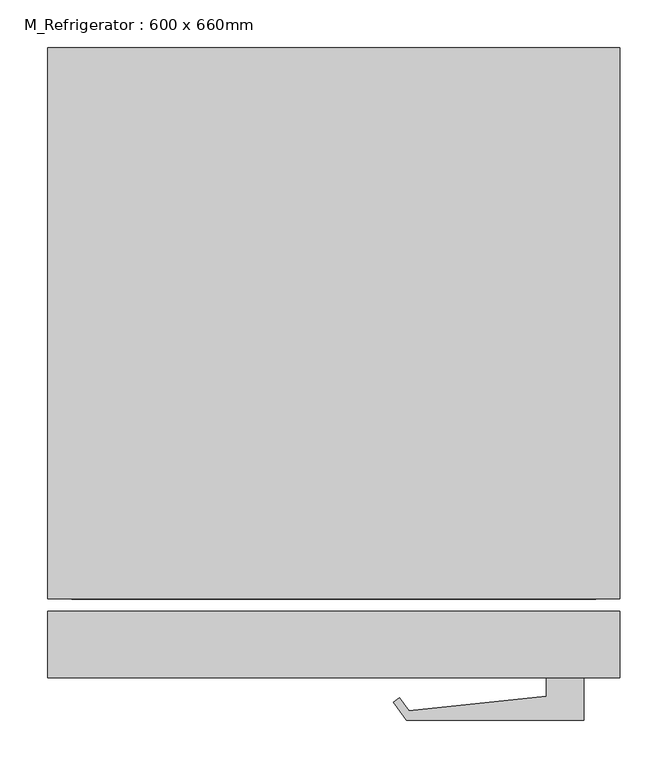
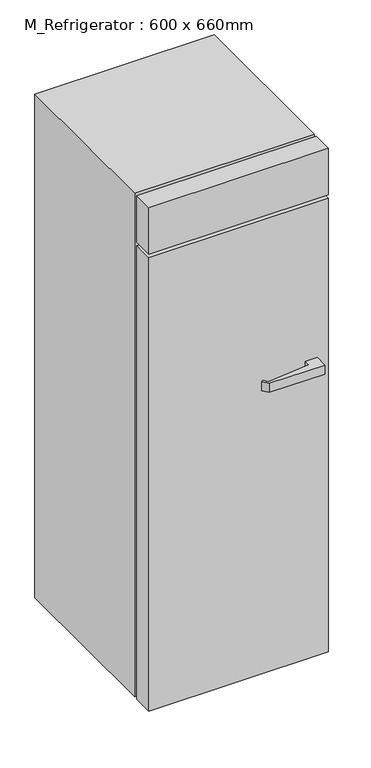
"""IFC4 building model written with IfcOpenShell, lengths in millimetres: proxy geometry, M_Refrigerator : 600 x 660mm."""

import ifcopenshell
import ifcopenshell.guid

model = None  # the IFC model being written
_history = None  # IfcOwnerHistory: only IFC2X3 demands one
_inside = {}  # id of a spatial element -> (the spatial element, [elements in it])
_under = {}  # id of a project, library or spatial element -> (it, [spatial elements below it])
_declared = {}  # id of a project -> (the project, [libraries it declares])
_typed = {}  # id of a type object -> (the type object, [elements of that type])
_made_of = {}  # id of a material, layer set ... -> (it, [elements and type objects made of it])


def new_model(schema):
    """Start an empty IFC model of exactly this schema.

    Asked for "IFC4X3", IfcOpenShell would pick the latest addendum, in which some entities
    have other attributes; the version numbers below select the first issue.
    IFC2X3 requires an IfcOwnerHistory on every rooted entity: one is made here for all.
    """
    global model, _history
    if schema == "IFC4X3":
        model = ifcopenshell.file(schema_version=(4, 3, 0, 0))
    else:
        model = ifcopenshell.file(schema=schema)
    _inside.clear()
    _under.clear()
    _declared.clear()
    _typed.clear()
    _made_of.clear()
    _history = None
    if model.schema == "IFC2X3":
        org = make("IfcOrganization", Name="unknown")
        user = make(
            "IfcPersonAndOrganization",
            ThePerson=make("IfcPerson", FamilyName="unknown"),
            TheOrganization=org,
        )
        app = make(
            "IfcApplication",
            ApplicationDeveloper=org,
            Version="unknown",
            ApplicationFullName="unknown",
            ApplicationIdentifier="unknown",
        )
        _history = make(
            "IfcOwnerHistory",
            OwningUser=user,
            OwningApplication=app,
            ChangeAction="ADDED",
            CreationDate=0,
        )
    return model


def make(cls, **values):
    """One entity of the class cls with the attributes given. An attribute that is None is left unset."""
    return model.create_entity(
        cls, **{name: value for name, value in values.items() if value is not None}
    )


def rooted(cls, **values):
    """An entity with a GlobalId (a new one), such as an element, a storey or a relation."""
    return make(cls, GlobalId=ifcopenshell.guid.new(), OwnerHistory=_history, **values)


def si_unit(unit_type, name, prefix=None):
    """IfcSIUnit, for example si_unit("LENGTHUNIT", "METRE", prefix="MILLI")."""
    return make("IfcSIUnit", UnitType=unit_type, Prefix=prefix, Name=name)


def assignment(units):
    """IfcUnitAssignment: the units of a project."""
    return None if units is None else make("IfcUnitAssignment", Units=units)


def point(xyz):
    """IfcCartesianPoint."""
    return None if xyz is None else make("IfcCartesianPoint", Coordinates=xyz)


def direction(xyz):
    """IfcDirection."""
    return None if xyz is None else make("IfcDirection", DirectionRatios=xyz)


def frame(location, z_axis=None, x_axis=None):
    """IfcAxis2Placement3D, a coordinate frame: its origin and axes. An axis left out is left unset."""
    return make(
        "IfcAxis2Placement3D",
        Location=point(location),
        Axis=direction(z_axis),
        RefDirection=direction(x_axis),
    )


def frame_2d(location, x_axis=None):
    """IfcAxis2Placement2D, a coordinate frame in the plane: its origin and x axis."""
    return make(
        "IfcAxis2Placement2D", Location=point(location), RefDirection=direction(x_axis)
    )


def origin():
    """The frame at (0, 0, 0) with its axes left unset."""
    return frame((0.0, 0.0, 0.0))


def origin_with_axes():
    """The frame at (0, 0, 0) with the z axis (0, 0, 1) and the x axis (1, 0, 0) written out."""
    return frame((0.0, 0.0, 0.0), z_axis=(0.0, 0.0, 1.0), x_axis=(1.0, 0.0, 0.0))


def place(relative_to, where):
    """IfcLocalPlacement: puts the frame where relative to a parent placement (None: the world)."""
    return make(
        "IfcLocalPlacement", PlacementRelTo=relative_to, RelativePlacement=where
    )


def context(
    kind, dimensions, precision=None, world=None, true_north=None, identifier=None
):
    """IfcGeometricRepresentationContext, for example the 3D "Model" context."""
    return make(
        "IfcGeometricRepresentationContext",
        ContextIdentifier=identifier,
        ContextType=kind,
        CoordinateSpaceDimension=dimensions,
        Precision=precision,
        WorldCoordinateSystem=world,
        TrueNorth=true_north,
    )


def project(units=None, contexts=None):
    """IfcProject with its units and contexts."""
    return rooted(
        "IfcProject",
        Name="project",
        RepresentationContexts=contexts,
        UnitsInContext=assignment(units),
    )


def spatial(cls, under=None, at=None, **own):
    """A site, building, storey or space (cls), placed at a placement, below another one or the project."""
    s = rooted(cls, ObjectPlacement=at, **own)
    if under is not None:
        _under.setdefault(under.id(), (under, []))[1].append(s)
    return s


def polyline(points):
    """IfcPolyline through the points."""
    return make("IfcPolyline", Points=[point(p) for p in points])


def circle_curve(where, radius):
    """IfcCircle in the frame where."""
    return make("IfcCircle", Position=where, Radius=radius)


def trimmed(basis, trim1, trim2, sense, master):
    """IfcTrimmedCurve: the piece of a basis curve between two trims."""
    return make(
        "IfcTrimmedCurve",
        BasisCurve=basis,
        Trim1=trim1,
        Trim2=trim2,
        SenseAgreement=sense,
        MasterRepresentation=master,
    )


def segment(curve, same_sense, transition):
    """IfcCompositeCurveSegment."""
    return make(
        "IfcCompositeCurveSegment",
        Transition=transition,
        SameSense=same_sense,
        ParentCurve=curve,
    )


def composite_curve(segments, self_intersect=None):
    """IfcCompositeCurve: segments joined end to end."""
    return make("IfcCompositeCurve", Segments=segments, SelfIntersect=self_intersect)


def outline(outer, holes=None, kind="AREA"):
    """IfcArbitraryClosedProfileDef: a profile drawn as a closed curve; with holes, ...WithVoids."""
    if holes is None:
        return make("IfcArbitraryClosedProfileDef", ProfileType=kind, OuterCurve=outer)
    return make(
        "IfcArbitraryProfileDefWithVoids",
        ProfileType=kind,
        OuterCurve=outer,
        InnerCurves=holes,
    )


def extrude(swept, where, along, depth):
    """IfcExtrudedAreaSolid: the profile swept, set in the frame where, extruded along a direction by depth."""
    return make(
        "IfcExtrudedAreaSolid",
        SweptArea=swept,
        Position=where,
        ExtrudedDirection=direction(along),
        Depth=depth,
    )


def shape(context_of_items, identifier, shape_type, items):
    """IfcShapeRepresentation: the items that make up one representation, for example the "Body"."""
    return make(
        "IfcShapeRepresentation",
        ContextOfItems=context_of_items,
        RepresentationIdentifier=identifier,
        RepresentationType=shape_type,
        Items=items,
    )


def source(mapping_origin, context_of_items, identifier, shape_type, items):
    """IfcRepresentationMap: a shape defined once, which mapped items show again and again."""
    return make(
        "IfcRepresentationMap",
        MappingOrigin=mapping_origin,
        MappedRepresentation=shape(context_of_items, identifier, shape_type, items),
    )


def transform(
    local_origin,
    x_axis=None,
    y_axis=None,
    z_axis=None,
    scale=None,
    scale2=None,
    scale3=None,
    uniform=True,
):
    """IfcCartesianTransformationOperator3D, or its non-uniform kind. x_axis, y_axis, z_axis: its Axis1, 2, 3."""
    if uniform:
        return make(
            "IfcCartesianTransformationOperator3D",
            Axis1=direction(x_axis),
            Axis2=direction(y_axis),
            LocalOrigin=point(local_origin),
            Scale=scale,
            Axis3=direction(z_axis),
        )
    return make(
        "IfcCartesianTransformationOperator3DnonUniform",
        Axis1=direction(x_axis),
        Axis2=direction(y_axis),
        LocalOrigin=point(local_origin),
        Scale=scale,
        Axis3=direction(z_axis),
        Scale2=scale2,
        Scale3=scale3,
    )


def mapped(mapping_source, mapping_target):
    """IfcMappedItem: shows the shape of a source again, moved by a transform."""
    return make(
        "IfcMappedItem", MappingSource=mapping_source, MappingTarget=mapping_target
    )


def made_of(thing, what):
    """Note that an element or type object is made of a material, layer set ...; save() writes the relation."""
    if what is not None:
        _made_of.setdefault(what.id(), (what, []))[1].append(thing)
    return thing


def element(
    cls,
    number,
    at=None,
    inside=None,
    cuts=None,
    type_object=None,
    material=None,
    context=None,
    identifier="Body",
    shape_type=None,
    held_by="IfcProductDefinitionShape",
    body=None,
    shapes=None,
    **own,
):
    """One element of the class cls, such as IfcWall. Its Tag is "e" and its number.

    at: its placement. inside: the storey or other place that contains it. cuts: it is an
    opening in that element (IfcRelVoidsElement). A single representation is given by context,
    identifier, shape_type and body (its items); several are given by shapes. held_by: the class
    of the entity that holds the representations. save() writes the other relations.
    """
    e = rooted(cls, Tag="e%d" % number, ObjectPlacement=at, **own)
    if body is not None:
        shapes = [shape(context, identifier, shape_type, body)]
    if shapes is not None:
        e.Representation = make(held_by, Representations=shapes)
    if inside is not None:
        _inside.setdefault(inside.id(), (inside, []))[1].append(e)
    if cuts is not None:
        rooted(
            "IfcRelVoidsElement", RelatingBuildingElement=cuts, RelatedOpeningElement=e
        )
    if type_object is not None:
        _typed.setdefault(type_object.id(), (type_object, []))[1].append(e)
    return made_of(e, material)


def aggregate(whole, parts):
    """IfcRelAggregates: a whole, such as a stair, and the parts it consists of."""
    return rooted("IfcRelAggregates", RelatingObject=whole, RelatedObjects=parts)


def save(model, path):
    """Write the relations noted so far, then the file.

    IfcRelAggregates (storeys below a building ...), IfcRelContainedInSpatialStructure (elements
    in a storey), IfcRelDefinesByType, IfcRelAssociatesMaterial and IfcRelDeclares: one each for
    every whole, place, type object, material and project.
    """
    for whole, parts in _under.values():
        aggregate(whole, parts)
    for where, things in _inside.values():
        rooted(
            "IfcRelContainedInSpatialStructure",
            RelatedElements=things,
            RelatingStructure=where,
        )
    for kind, things in _typed.values():
        rooted("IfcRelDefinesByType", RelatedObjects=things, RelatingType=kind)
    for what, things in _made_of.values():
        rooted("IfcRelAssociatesMaterial", RelatedObjects=things, RelatingMaterial=what)
    for by, libraries in _declared.values():
        rooted("IfcRelDeclares", RelatingContext=by, RelatedDefinitions=libraries)
    model.write(path)


def m_refrigerator_600_x_660mm_a466bf94(model_context):
    return source(origin(), model_context, "Body", "SweptSolid", [
        extrude(outline(polyline([(208.0988574, -408.1036861), (22.3988574, -408.1036861), (8.7240737, -389.5368406), (15.2273026, -384.7471068), (25.1756383, -398.2543926), (168.9242419, -383.0358618), (168.9242419, -363.7849098), (208.0988574, -363.7849098), (208.0988574, -408.1036861)])), frame((0.0, 0.0, 1071.927792), z_axis=(0.0, 0.0, 1.0), x_axis=(1.0, 0.0, 0.0)), (0.0, 0.0, 1.0), 31.75),
        extrude(outline(composite_curve([segment(trimmed(circle_curve(frame_2d((-271.2511426, 220.0150902)), 25.4), [point((-296.6511426, 220.0150902))], [point((-245.8511426, 220.0150902))], False, "CARTESIAN"), True, "CONTINUOUS"), segment(trimmed(circle_curve(frame_2d((-271.2511426, 220.0150902)), 25.4), [point((-245.8511426, 220.0150902))], [point((-296.6511426, 220.0150902))], False, "CARTESIAN"), True, "CONTINUOUS")], self_intersect=False)), origin_with_axes(), (0.0, 0.0, 1.0), 50.8),
        extrude(outline(composite_curve([segment(trimmed(circle_curve(frame_2d((163.6488574, 220.0150902)), 25.4), [point((138.2488574, 220.0150902))], [point((189.0488574, 220.0150902))], False, "CARTESIAN"), True, "CONTINUOUS"), segment(trimmed(circle_curve(frame_2d((163.6488574, 220.0150902)), 25.4), [point((189.0488574, 220.0150902))], [point((138.2488574, 220.0150902))], False, "CARTESIAN"), True, "CONTINUOUS")], self_intersect=False)), origin_with_axes(), (0.0, 0.0, 1.0), 50.8),
        extrude(outline(composite_curve([segment(trimmed(circle_curve(frame_2d((-271.2511426, -236.7849098)), 25.4), [point((-296.6511426, -236.7849098))], [point((-245.8511426, -236.7849098))], False, "CARTESIAN"), True, "CONTINUOUS"), segment(trimmed(circle_curve(frame_2d((-271.2511426, -236.7849098)), 25.4), [point((-245.8511426, -236.7849098))], [point((-296.6511426, -236.7849098))], False, "CARTESIAN"), True, "CONTINUOUS")], self_intersect=False)), origin_with_axes(), (0.0, 0.0, 1.0), 50.8),
        extrude(outline(composite_curve([segment(trimmed(circle_curve(frame_2d((163.6488574, -236.7849098)), 25.4), [point((138.2488574, -236.7849098))], [point((189.0488574, -236.7849098))], False, "CARTESIAN"), True, "CONTINUOUS"), segment(trimmed(circle_curve(frame_2d((163.6488574, -236.7849098)), 25.4), [point((189.0488574, -236.7849098))], [point((138.2488574, -236.7849098))], False, "CARTESIAN"), True, "CONTINUOUS")], self_intersect=False)), origin_with_axes(), (0.0, 0.0, 1.0), 50.8),
        extrude(outline(polyline([(246.1988574, -363.7849098), (-353.8011426, -363.7849098), (-353.8011426, -293.9349098), (246.1988574, -293.9349098), (246.1988574, -363.7849098)])), frame((0.0, 0.0, 50.8), z_axis=(0.0, 0.0, 1.0), x_axis=(1.0, 0.0, 0.0)), (0.0, 0.0, 1.0), 1601.4),
        extrude(outline(polyline([(246.1988574, -363.7849098), (-353.8011426, -363.7849098), (-353.8011426, -293.9349098), (246.1988574, -293.9349098), (246.1988574, -363.7849098)])), frame((0.0, 0.0, 1664.9), z_axis=(0.0, 0.0, 1.0), x_axis=(1.0, 0.0, 0.0)), (0.0, 0.0, 1.0), 165.1),
        extrude(outline(polyline([(220.7988574, 270.8150902), (-328.4011426, 270.8150902), (-328.4011426, 296.2150902), (220.7988574, 296.2150902), (220.7988574, 270.8150902)])), frame((0.0, 0.0, 152.4), z_axis=(0.0, 0.0, 1.0), x_axis=(1.0, 0.0, 0.0)), (0.0, 0.0, 1.0), 1652.2),
        extrude(outline(polyline([(1830.0, 246.1988574), (1830.0, -353.8011426), (50.8, -353.8011426), (50.8, 246.1988574), (1830.0, 246.1988574)]), holes=[polyline([(1626.8, 220.7988574), (431.8, 220.7988574), (431.8, -328.4011426), (1626.8, -328.4011426), (1626.8, 220.7988574)])]), frame((0.0, -281.2349098, 0.0), z_axis=(0.0, 1.0, 0.0), x_axis=(0.0, 0.0, 1.0)), (0.0, 0.0, 1.0), 577.45),
    ])


if __name__ == "__main__":
    model = new_model("IFC4")
    model_context = context("Model", 3, world=origin())
    ifc_project = project(units=[si_unit("LENGTHUNIT", "METRE", prefix="MILLI")], contexts=[model_context])
    site = spatial("IfcSite", under=ifc_project)
    building = spatial("IfcBuilding", under=site)
    placement = place(None, origin())
    m_refrigerator_600_x_660mm_shape = m_refrigerator_600_x_660mm_a466bf94(model_context)
    element("IfcBuildingElementProxy", 1, Name="M_Refrigerator : 600 x 660mm", ObjectType="M_Refrigerator : 600 x 660mm", at=placement, inside=building, context=model_context, shape_type="MappedRepresentation", body=[
        mapped(m_refrigerator_600_x_660mm_shape, transform((0.0, 0.0, 0.0), x_axis=(1.0, 0.0, 0.0), y_axis=(0.0, 1.0, 0.0), z_axis=(0.0, 0.0, 1.0))),
    ])
    save(model, "model.ifc")

# Revit data of these elements
# Type "M_Refrigerator : 600 x 660mm"
#   Type IfcGUID = "095ehmSozDWfEWYyuf2xS6"
#   Label = "REF."
#   Depth = 660 mm
#   Height = 1830 mm
#   Width = 600 mm
#   Material = Steel, Paint Finish, Ivory, Matte
#   Description = (empty or 0)
#   Default Elevation = 0
# Element 1 (IfcBuildingElementProxy, "M_Refrigerator : 600 x 660mm")
#   Materials on its faces: "Steel, Paint Finish, Ivory, Matte", "Steel, Chrome Plated"
# Materials
#   "Steel, Paint Finish, Ivory, Matte": class "Metal", colour RGB 247 247 239, transparency 0, Description = "Steel, paint finish, ivory, matte", Cost = 0
#   "Steel, Chrome Plated": class "Metal", colour RGB 120 120 120, transparency 0, Description = "Chromiuim plated steel", Cost = 0
